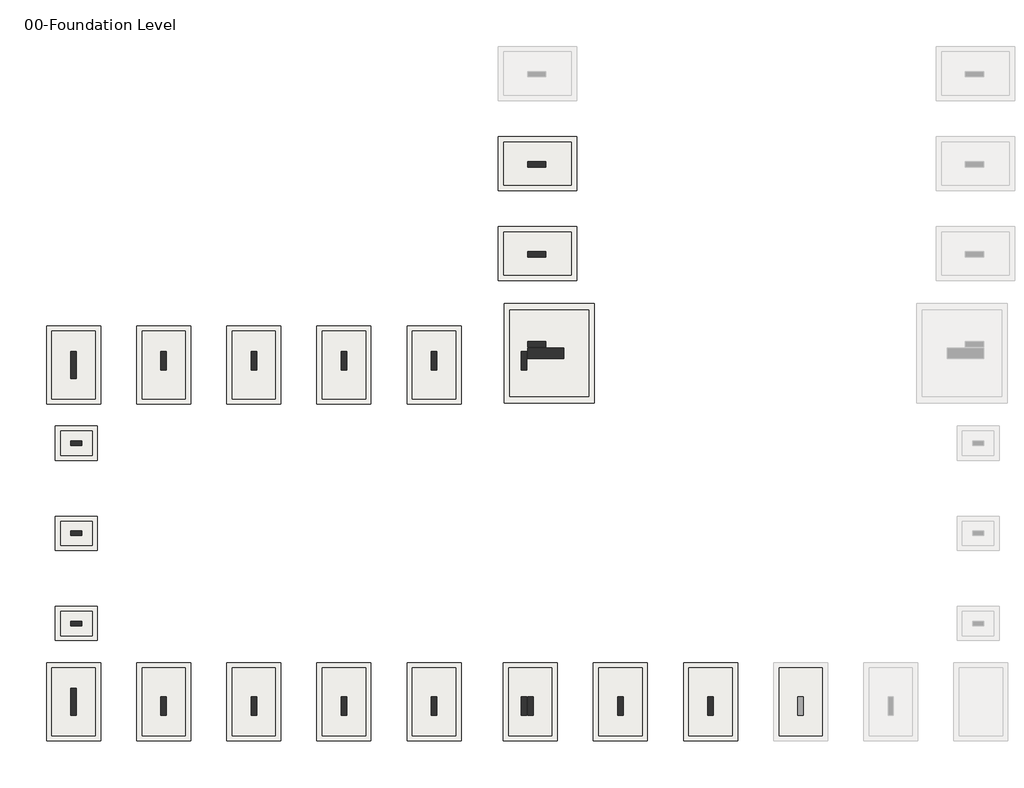
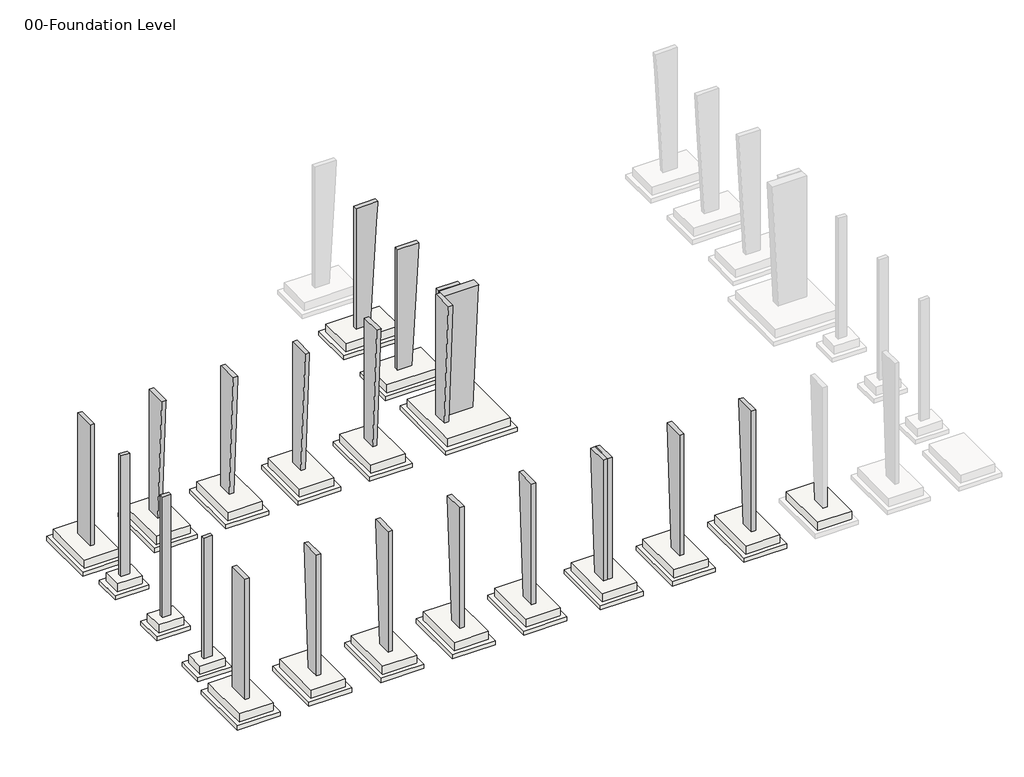
# One storey, part 1 of 4: 39 slabs, 22 columns.
"""IFC4 building model written with IfcOpenShell, lengths in millimetres."""

import ifcopenshell
import ifcopenshell.guid

model = None  # the IFC model being written
_history = None  # IfcOwnerHistory: only IFC2X3 demands one
_inside = {}  # id of a spatial element -> (the spatial element, [elements in it])
_under = {}  # id of a project, library or spatial element -> (it, [spatial elements below it])
_declared = {}  # id of a project -> (the project, [libraries it declares])
_typed = {}  # id of a type object -> (the type object, [elements of that type])
_made_of = {}  # id of a material, layer set ... -> (it, [elements and type objects made of it])


def new_model(schema):
    """Start an empty IFC model of exactly this schema.

    Asked for "IFC4X3", IfcOpenShell would pick the latest addendum, in which some entities
    have other attributes; the version numbers below select the first issue.
    IFC2X3 requires an IfcOwnerHistory on every rooted entity: one is made here for all.
    """
    global model, _history
    if schema == "IFC4X3":
        model = ifcopenshell.file(schema_version=(4, 3, 0, 0))
    else:
        model = ifcopenshell.file(schema=schema)
    _inside.clear()
    _under.clear()
    _declared.clear()
    _typed.clear()
    _made_of.clear()
    _history = None
    if model.schema == "IFC2X3":
        org = make("IfcOrganization", Name="unknown")
        user = make(
            "IfcPersonAndOrganization",
            ThePerson=make("IfcPerson", FamilyName="unknown"),
            TheOrganization=org,
        )
        app = make(
            "IfcApplication",
            ApplicationDeveloper=org,
            Version="unknown",
            ApplicationFullName="unknown",
            ApplicationIdentifier="unknown",
        )
        _history = make(
            "IfcOwnerHistory",
            OwningUser=user,
            OwningApplication=app,
            ChangeAction="ADDED",
            CreationDate=0,
        )
    return model


def make(cls, **values):
    """One entity of the class cls with the attributes given. An attribute that is None is left unset."""
    return model.create_entity(
        cls, **{name: value for name, value in values.items() if value is not None}
    )


def rooted(cls, **values):
    """An entity with a GlobalId (a new one), such as an element, a storey or a relation."""
    return make(cls, GlobalId=ifcopenshell.guid.new(), OwnerHistory=_history, **values)


def si_unit(unit_type, name, prefix=None):
    """IfcSIUnit, for example si_unit("LENGTHUNIT", "METRE", prefix="MILLI")."""
    return make("IfcSIUnit", UnitType=unit_type, Prefix=prefix, Name=name)


def assignment(units):
    """IfcUnitAssignment: the units of a project."""
    return None if units is None else make("IfcUnitAssignment", Units=units)


def point(xyz):
    """IfcCartesianPoint."""
    return None if xyz is None else make("IfcCartesianPoint", Coordinates=xyz)


def direction(xyz):
    """IfcDirection."""
    return None if xyz is None else make("IfcDirection", DirectionRatios=xyz)


def frame(location, z_axis=None, x_axis=None):
    """IfcAxis2Placement3D, a coordinate frame: its origin and axes. An axis left out is left unset."""
    return make(
        "IfcAxis2Placement3D",
        Location=point(location),
        Axis=direction(z_axis),
        RefDirection=direction(x_axis),
    )


def origin():
    """The frame at (0, 0, 0) with its axes left unset."""
    return frame((0.0, 0.0, 0.0))


def place(relative_to, where):
    """IfcLocalPlacement: puts the frame where relative to a parent placement (None: the world)."""
    return make(
        "IfcLocalPlacement", PlacementRelTo=relative_to, RelativePlacement=where
    )


def context(
    kind, dimensions, precision=None, world=None, true_north=None, identifier=None
):
    """IfcGeometricRepresentationContext, for example the 3D "Model" context."""
    return make(
        "IfcGeometricRepresentationContext",
        ContextIdentifier=identifier,
        ContextType=kind,
        CoordinateSpaceDimension=dimensions,
        Precision=precision,
        WorldCoordinateSystem=world,
        TrueNorth=true_north,
    )


def project(units=None, contexts=None):
    """IfcProject with its units and contexts."""
    return rooted(
        "IfcProject",
        Name="project",
        RepresentationContexts=contexts,
        UnitsInContext=assignment(units),
    )


def spatial(cls, under=None, at=None, **own):
    """A site, building, storey or space (cls), placed at a placement, below another one or the project."""
    s = rooted(cls, ObjectPlacement=at, **own)
    if under is not None:
        _under.setdefault(under.id(), (under, []))[1].append(s)
    return s


def polyline(points):
    """IfcPolyline through the points."""
    return make("IfcPolyline", Points=[point(p) for p in points])


def outline(outer, holes=None, kind="AREA"):
    """IfcArbitraryClosedProfileDef: a profile drawn as a closed curve; with holes, ...WithVoids."""
    if holes is None:
        return make("IfcArbitraryClosedProfileDef", ProfileType=kind, OuterCurve=outer)
    return make(
        "IfcArbitraryProfileDefWithVoids",
        ProfileType=kind,
        OuterCurve=outer,
        InnerCurves=holes,
    )


def extrude(swept, where, along, depth):
    """IfcExtrudedAreaSolid: the profile swept, set in the frame where, extruded along a direction by depth."""
    return make(
        "IfcExtrudedAreaSolid",
        SweptArea=swept,
        Position=where,
        ExtrudedDirection=direction(along),
        Depth=depth,
    )


def faces_of(points, faces, orient=None, outer=None):
    """IfcFace entities. A face is a list of loops; a loop is a list of indices into points, from 0.

    orient and outer hold one flag for each loop. By default every Orientation is true, the
    first loop of a face is its IfcFaceOuterBound and the others are IfcFaceBound.
    """
    made = []
    for i, loops in enumerate(faces):
        bounds = []
        for j, loop in enumerate(loops):
            is_outer = j == 0 if outer is None else outer[i][j]
            bounds.append(
                make(
                    "IfcFaceOuterBound" if is_outer else "IfcFaceBound",
                    Bound=make("IfcPolyLoop", Polygon=[points[k] for k in loop]),
                    Orientation=True if orient is None else orient[i][j],
                )
            )
        made.append(make("IfcFace", Bounds=bounds))
    return made


def faceted_brep(points, faces, orient=None, outer=None, voids=None):
    """IfcFacetedBrep: a solid bounded by flat faces; with voids (closed shells), ...WithVoids."""
    shared = [point(p) for p in points]
    hull = make("IfcClosedShell", CfsFaces=faces_of(shared, faces, orient, outer))
    if voids is None:
        return make("IfcFacetedBrep", Outer=hull)
    return make(
        "IfcFacetedBrepWithVoids",
        Outer=hull,
        Voids=[
            make(cls, CfsFaces=faces_of(shared, fs, o, b)) for cls, fs, o, b in voids
        ],
    )


def shape(context_of_items, identifier, shape_type, items):
    """IfcShapeRepresentation: the items that make up one representation, for example the "Body"."""
    return make(
        "IfcShapeRepresentation",
        ContextOfItems=context_of_items,
        RepresentationIdentifier=identifier,
        RepresentationType=shape_type,
        Items=items,
    )


def made_of(thing, what):
    """Note that an element or type object is made of a material, layer set ...; save() writes the relation."""
    if what is not None:
        _made_of.setdefault(what.id(), (what, []))[1].append(thing)
    return thing


def element(
    cls,
    number,
    at=None,
    inside=None,
    cuts=None,
    type_object=None,
    material=None,
    context=None,
    identifier="Body",
    shape_type=None,
    held_by="IfcProductDefinitionShape",
    body=None,
    shapes=None,
    **own,
):
    """One element of the class cls, such as IfcWall. Its Tag is "e" and its number.

    at: its placement. inside: the storey or other place that contains it. cuts: it is an
    opening in that element (IfcRelVoidsElement). A single representation is given by context,
    identifier, shape_type and body (its items); several are given by shapes. held_by: the class
    of the entity that holds the representations. save() writes the other relations.
    """
    e = rooted(cls, Tag="e%d" % number, ObjectPlacement=at, **own)
    if body is not None:
        shapes = [shape(context, identifier, shape_type, body)]
    if shapes is not None:
        e.Representation = make(held_by, Representations=shapes)
    if inside is not None:
        _inside.setdefault(inside.id(), (inside, []))[1].append(e)
    if cuts is not None:
        rooted(
            "IfcRelVoidsElement", RelatingBuildingElement=cuts, RelatedOpeningElement=e
        )
    if type_object is not None:
        _typed.setdefault(type_object.id(), (type_object, []))[1].append(e)
    return made_of(e, material)


def aggregate(whole, parts):
    """IfcRelAggregates: a whole, such as a stair, and the parts it consists of."""
    return rooted("IfcRelAggregates", RelatingObject=whole, RelatedObjects=parts)


def save(model, path):
    """Write the relations noted so far, then the file.

    IfcRelAggregates (storeys below a building ...), IfcRelContainedInSpatialStructure (elements
    in a storey), IfcRelDefinesByType, IfcRelAssociatesMaterial and IfcRelDeclares: one each for
    every whole, place, type object, material and project.
    """
    for whole, parts in _under.values():
        aggregate(whole, parts)
    for where, things in _inside.values():
        rooted(
            "IfcRelContainedInSpatialStructure",
            RelatedElements=things,
            RelatingStructure=where,
        )
    for kind, things in _typed.values():
        rooted("IfcRelDefinesByType", RelatedObjects=things, RelatingType=kind)
    for what, things in _made_of.values():
        rooted("IfcRelAssociatesMaterial", RelatedObjects=things, RelatingMaterial=what)
    for by, libraries in _declared.values():
        rooted("IfcRelDeclares", RelatingContext=by, RelatedDefinitions=libraries)
    model.write(path)


model = new_model("IFC4")

# Units and contexts
model_context = context("Model", 3, world=origin())
ifc_project = project(units=[si_unit("LENGTHUNIT", "METRE", prefix="MILLI")], contexts=[model_context])

# Site, building, storey
site = spatial("IfcSite", under=ifc_project)
building = spatial("IfcBuilding", under=site)
storey = spatial("IfcBuildingStorey", under=building, Name="00-Foundation Level", Elevation=-2000.0)

# Columns
placement = place(None, origin())
element("IfcColumn", 1, ObjectType="Frame Col.2 : 1500x300", at=placement, inside=storey, context=model_context, shape_type="Brep", body=[
    faceted_brep([(25143.2245521, 19099.7448193, -1100.0), (25143.2245521, 20099.7448193, -1100.0), (25143.2245521, 20099.7448193, 7800.0), (25143.2245521, 18599.7448193, 7800.0), (25143.2245521, 18606.4863924, 7680.0), (24843.2245521, 18599.7448193, 7800.0), (24843.2245521, 18606.4863924, 7680.0), (24843.2245521, 19099.7448193, -1100.0), (24843.2245521, 20099.7448193, -1100.0), (24843.2245521, 20089.7085236, 7800.0), (24843.2245521, 20099.7448193, 7800.0)], [[[0, 1, 2, 3, 4]], [[0, 4, 3, 5, 6, 7]], [[8, 7, 6, 5, 9, 10]], [[2, 1, 8, 10]], [[1, 0, 7, 8]], [[3, 2, 10, 9, 5]]]),
])
element("IfcColumn", 2, ObjectType="Frame Col.2 : 1500x300", at=placement, inside=storey, context=model_context, shape_type="Brep", body=[
    faceted_brep([(20143.2245522, 19099.7448193, -1100.0), (20143.2245522, 20099.7448193, -1100.0), (20143.2245522, 20099.7448193, 7800.0), (20143.2245522, 20089.7085236, 7800.0), (20143.2245522, 18599.7448193, 7800.0), (20143.2245522, 18606.4863924, 7680.0), (19843.2245522, 18599.7448193, 7800.0), (19843.2245522, 18606.4863924, 7680.0), (19843.2245522, 19099.7448193, -1100.0), (19843.2245522, 20099.7448193, -1100.0), (19843.2245522, 20089.7085236, 7800.0), (19843.2245522, 20099.7448193, 7800.0)], [[[0, 1, 2, 3, 4, 5]], [[0, 5, 4, 6, 7, 8]], [[9, 8, 7, 6, 10, 11]], [[2, 1, 9, 11]], [[1, 0, 8, 9]], [[4, 3, 2, 11, 10, 6]]]),
])
element("IfcColumn", 3, ObjectType="Frame Col.2 : 1500x300", at=placement, inside=storey, context=model_context, shape_type="Brep", body=[
    faceted_brep([(15143.2245516, 19099.7448193, -1100.0), (15143.2245516, 20099.7448193, -1100.0), (15143.2245516, 20099.7448193, 7800.0), (15143.2245516, 20089.7085236, 7800.0), (15143.2245516, 18599.7448193, 7800.0), (15143.2245516, 18606.4863924, 7680.0), (14843.2245516, 18599.7448193, 7800.0), (14843.2245516, 18606.4863924, 7680.0), (14843.2245516, 19099.7448193, -1100.0), (14843.2245516, 20099.7448193, -1100.0), (14843.2245516, 20089.7085236, 7800.0), (14843.2245516, 20099.7448193, 7800.0)], [[[0, 1, 2, 3, 4, 5]], [[0, 5, 4, 6, 7, 8]], [[9, 8, 7, 6, 10, 11]], [[2, 1, 9, 11]], [[1, 0, 8, 9]], [[4, 3, 2, 11, 10, 6]]]),
])
element("IfcColumn", 4, ObjectType="Frame Col.2 : 1500x300", at=placement, inside=storey, context=model_context, shape_type="Brep", body=[
    faceted_brep([(10143.2245521, 19099.7448193, -1100.0), (10143.2245521, 20099.7448193, -1100.0), (10143.2245521, 20099.7448193, 7800.0), (10143.2245521, 20089.7085236, 7800.0), (10143.2245521, 18599.7448193, 7800.0), (10143.2245521, 18606.4863924, 7680.0), (9843.2245521, 18599.7448193, 7800.0), (9843.2245521, 18606.4863924, 7680.0), (9843.2245521, 19099.7448193, -1100.0), (9843.2245521, 20099.7448193, -1100.0), (9843.2245521, 20089.7085236, 7800.0), (9843.2245521, 20099.7448193, 7800.0)], [[[0, 1, 2, 3, 4, 5]], [[0, 5, 4, 6, 7, 8]], [[9, 8, 7, 6, 10, 11]], [[2, 1, 9, 11]], [[1, 0, 8, 9]], [[4, 3, 2, 11, 10, 6]]]),
])
element("IfcColumn", 5, ObjectType="Frame Col.2 : 1500x300", at=placement, inside=storey, context=model_context, shape_type="Brep", body=[
    faceted_brep([(5143.2245516, 19099.7448193, -1100.0), (5143.2245516, 20099.7448193, -1100.0), (5143.2245516, 20099.7448193, 7800.0), (5143.2245516, 20089.7085236, 7800.0), (5143.2245516, 18599.7448193, 7800.0), (5143.2245516, 18606.4863924, 7680.0), (4843.2245516, 18599.7448193, 7800.0), (4843.2245516, 18606.4863924, 7680.0), (4843.2245516, 19099.7448193, -1100.0), (4843.2245516, 20099.7448193, -1100.0), (4843.2245516, 20089.7085236, 7800.0), (4843.2245516, 20099.7448193, 7800.0)], [[[0, 1, 2, 3, 4, 5]], [[0, 5, 4, 6, 7, 8]], [[9, 8, 7, 6, 10, 11]], [[2, 1, 9, 11]], [[1, 0, 8, 9]], [[4, 3, 2, 11, 10, 6]]]),
])
element("IfcColumn", 6, ObjectType="Frame Col.2 : 1500x300", at=placement, inside=storey, context=model_context, shape_type="Brep", body=[
    faceted_brep([(30183.2245515, 899.7448196, -1100.0), (30183.2245515, -100.2551804, -1100.0), (30183.2245515, -100.2551804, 7680.0), (30183.2245515, -100.2551804, 7800.0), (30183.2245515, 1399.7448196, 7800.0), (30183.2245515, 1393.0032466, 7680.0), (30483.2245515, 1399.7448196, 7800.0), (30483.2245515, 1393.0032466, 7680.0), (30483.2245515, 899.7448196, -1100.0), (30483.2245515, -100.2551804, -1100.0), (30483.2245515, -100.2551804, 7800.0), (30483.2245515, -100.2551804, 7680.0)], [[[0, 1, 2, 3, 4, 5]], [[0, 5, 4, 6, 7, 8]], [[9, 8, 7, 6, 10, 11]], [[3, 2, 1, 9, 11, 10]], [[1, 0, 8, 9]], [[4, 3, 10, 6]]]),
])
element("IfcColumn", 7, ObjectType="Frame Col.2 : 1500x300", at=placement, inside=storey, context=model_context, shape_type="Brep", body=[
    faceted_brep([(25183.2245516, 899.7448196, -1100.0), (25183.2245516, -100.2551804, -1100.0), (25183.2245516, -100.2551804, 7800.0), (25183.2245516, 1399.7448196, 7800.0), (25183.2245516, 1393.0032466, 7680.0), (25483.2245516, 1399.7448196, 7800.0), (25483.2245516, 1393.0032466, 7680.0), (25483.2245516, 899.7448196, -1100.0), (25483.2245516, -100.2551804, -1100.0), (25483.2245516, -100.2551804, 7800.0), (25483.2245516, -100.2551804, 7680.0)], [[[0, 1, 2, 3, 4]], [[0, 4, 3, 5, 6, 7]], [[8, 7, 6, 5, 9, 10]], [[2, 1, 8, 10, 9]], [[1, 0, 7, 8]], [[3, 2, 9, 5]]]),
])
element("IfcColumn", 8, ObjectType="Frame Col.2 : 1500x300", at=placement, inside=storey, context=model_context, shape_type="Brep", body=[
    faceted_brep([(24843.2245521, 899.7448196, -1100.0), (24843.2245521, -100.2551804, -1100.0), (24843.2245521, -100.2551804, 7680.0), (24843.2245521, -100.2551804, 7800.0), (24843.2245521, 1399.7448196, 7800.0), (24843.2245521, 1393.0032466, 7680.0), (25143.2245521, 1399.7448196, 7800.0), (25143.2245521, 1393.0032466, 7680.0), (25143.2245521, 899.7448196, -1100.0), (25143.2245521, -100.2551804, -1100.0), (25143.2245521, -100.2551804, 7800.0), (25143.2245521, -100.2551804, 7680.0)], [[[0, 1, 2, 3, 4, 5]], [[0, 5, 4, 6, 7, 8]], [[9, 8, 7, 6, 10, 11]], [[3, 2, 1, 9, 11, 10]], [[1, 0, 8, 9]], [[4, 3, 10, 6]]]),
])
element("IfcColumn", 9, ObjectType="Frame Col.2 : 1500x300", at=placement, inside=storey, context=model_context, shape_type="Brep", body=[
    faceted_brep([(19843.2245522, 899.7448196, -1100.0), (19843.2245522, -100.2551804, -1100.0), (19843.2245522, -100.2551804, 7680.0), (19843.2245522, -100.2551804, 7800.0), (19843.2245522, 1399.7448196, 7800.0), (19843.2245522, 1393.0032466, 7680.0), (20143.2245522, 1399.7448196, 7800.0), (20143.2245522, 1393.0032466, 7680.0), (20143.2245522, 899.7448196, -1100.0), (20143.2245522, -100.2551804, -1100.0), (20143.2245522, -100.2551804, 7800.0), (20143.2245522, -100.2551804, 7680.0)], [[[0, 1, 2, 3, 4, 5]], [[0, 5, 4, 6, 7, 8]], [[9, 8, 7, 6, 10, 11]], [[3, 2, 1, 9, 11, 10]], [[1, 0, 8, 9]], [[4, 3, 10, 6]]]),
])
element("IfcColumn", 10, ObjectType="Frame Col.2 : 1500x300", at=placement, inside=storey, context=model_context, shape_type="Brep", body=[
    faceted_brep([(14843.2245516, 899.7448196, -1100.0), (14843.2245516, -100.2551804, -1100.0), (14843.2245516, -100.2551804, 7680.0), (14843.2245516, -100.2551804, 7800.0), (14843.2245516, 1399.7448196, 7800.0), (14843.2245516, 1393.0032466, 7680.0), (15143.2245516, 1399.7448196, 7800.0), (15143.2245516, 1393.0032466, 7680.0), (15143.2245516, 899.7448196, -1100.0), (15143.2245516, -100.2551804, -1100.0), (15143.2245516, -100.2551804, 7800.0), (15143.2245516, -100.2551804, 7680.0)], [[[0, 1, 2, 3, 4, 5]], [[0, 5, 4, 6, 7, 8]], [[9, 8, 7, 6, 10, 11]], [[3, 2, 1, 9, 11, 10]], [[1, 0, 8, 9]], [[4, 3, 10, 6]]]),
])
element("IfcColumn", 11, ObjectType="Frame Col.2 : 1500x300", at=placement, inside=storey, context=model_context, shape_type="Brep", body=[
    faceted_brep([(9843.2245521, 899.7448196, -1100.0), (9843.2245521, -100.2551804, -1100.0), (9843.2245521, -100.2551804, 7680.0), (9843.2245521, -100.2551804, 7800.0), (9843.2245521, 1399.7448196, 7800.0), (9843.2245521, 1393.0032466, 7680.0), (10143.2245521, 1399.7448196, 7800.0), (10143.2245521, 1393.0032466, 7680.0), (10143.2245521, 899.7448196, -1100.0), (10143.2245521, -100.2551804, -1100.0), (10143.2245521, -100.2551804, 7800.0), (10143.2245521, -100.2551804, 7680.0)], [[[0, 1, 2, 3, 4, 5]], [[0, 5, 4, 6, 7, 8]], [[9, 8, 7, 6, 10, 11]], [[3, 2, 1, 9, 11, 10]], [[1, 0, 8, 9]], [[4, 3, 10, 6]]]),
])
element("IfcColumn", 12, ObjectType="Frame Col.2 : 1500x300", at=placement, inside=storey, context=model_context, shape_type="Brep", body=[
    faceted_brep([(4843.2245516, 899.7448196, -1100.0), (4843.2245516, -100.2551804, -1100.0), (4843.2245516, -100.2551804, 7680.0), (4843.2245516, -100.2551804, 7800.0), (4843.2245516, 1399.7448196, 7800.0), (4843.2245516, 1393.0032466, 7680.0), (5143.2245516, 1399.7448196, 7800.0), (5143.2245516, 1393.0032466, 7680.0), (5143.2245516, 899.7448196, -1100.0), (5143.2245516, -100.2551804, -1100.0), (5143.2245516, -100.2551804, 7800.0), (5143.2245516, -100.2551804, 7680.0)], [[[0, 1, 2, 3, 4, 5]], [[0, 5, 4, 6, 7, 8]], [[9, 8, 7, 6, 10, 11]], [[3, 2, 1, 9, 11, 10]], [[1, 0, 8, 9]], [[4, 3, 10, 6]]]),
])
element("IfcColumn", 13, ObjectType="Frame Col.2 : 1500x300", at=placement, inside=storey, context=model_context, shape_type="Brep", body=[
    faceted_brep([(26183.2245516, 20639.9999998, -1100.0), (25183.2245516, 20639.9999998, -1100.0), (25183.2245516, 20639.9999998, 7680.0), (25183.2245516, 20639.9999998, 7800.0), (26683.2245516, 20639.9999998, 7800.0), (26676.4829785, 20639.9999998, 7680.0), (26683.2245516, 20339.9999998, 7800.0), (26676.4829785, 20339.9999998, 7680.0), (26183.2245516, 20339.9999998, -1100.0), (25183.2245516, 20339.9999998, -1100.0), (25183.2245516, 20339.9999998, 7800.0)], [[[0, 1, 2, 3, 4, 5]], [[0, 5, 4, 6, 7, 8]], [[9, 8, 7, 6, 10]], [[3, 2, 1, 9, 10]], [[1, 0, 8, 9]], [[4, 3, 10, 6]]]),
])
element("IfcColumn", 14, ObjectType="Frame Col.2 : 1500x300", at=placement, inside=storey, context=model_context, shape_type="Brep", body=[
    faceted_brep([(35183.2245515, 899.7448196, -1100.0), (35183.2245515, -100.2551804, -1100.0), (35183.2245515, -100.2551804, 7680.0), (35183.2245515, -100.2551804, 7800.0), (35183.2245515, 1399.7448196, 7800.0), (35183.2245515, 1393.0032466, 7680.0), (35483.2245515, 1399.7448196, 7800.0), (35483.2245515, 1393.0032466, 7680.0), (35483.2245515, 899.7448196, -1100.0), (35483.2245515, -100.2551804, -1100.0), (35483.2245515, -100.2551804, 7800.0), (35483.2245515, -100.2551804, 7680.0)], [[[0, 1, 2, 3, 4, 5]], [[0, 5, 4, 6, 7, 8]], [[9, 8, 7, 6, 10, 11]], [[3, 2, 1, 9, 11, 10]], [[1, 0, 8, 9]], [[4, 3, 10, 6]]]),
])
element("IfcColumn", 15, ObjectType="Frame Col.2 : 1500x300", at=placement, inside=storey, context=model_context, shape_type="Brep", body=[
    faceted_brep([(26183.2245516, 25639.9999988, -1100.0), (25183.2245516, 25639.9999988, -1100.0), (25183.2245516, 25639.9999988, 7680.0), (25183.2245516, 25639.9999988, 7800.0), (26683.2245516, 25639.9999988, 7800.0), (26676.4829785, 25639.9999988, 7680.0), (26598.9548887, 25639.9999988, 6300.0), (26683.2245516, 25339.9999988, 7800.0), (26676.4829785, 25339.9999988, 7680.0), (26598.9548887, 25339.9999988, 6300.0), (26183.2245516, 25339.9999988, -1100.0), (25183.2245516, 25339.9999988, -1100.0), (25183.2245516, 25339.9999988, 7800.0), (25183.2245516, 25339.9999988, 7680.0)], [[[0, 1, 2, 3, 4, 5, 6]], [[0, 6, 5, 4, 7, 8, 9, 10]], [[11, 10, 9, 8, 7, 12, 13]], [[3, 2, 1, 11, 13, 12]], [[1, 0, 10, 11]], [[4, 3, 12, 7]]]),
])
element("IfcColumn", 16, ObjectType="Frame Col.2 : 1500x300", at=placement, inside=storey, context=model_context, shape_type="Brep", body=[
    faceted_brep([(26183.2245516, 30639.9999988, -1100.0), (25183.2245516, 30639.9999988, -1100.0), (25183.2245516, 30639.9999988, 7680.0), (25183.2245516, 30639.9999988, 7800.0), (26683.2245516, 30639.9999988, 7800.0), (26676.4829785, 30639.9999988, 7680.0), (26598.9548887, 30639.9999988, 6300.0), (26683.2245516, 30339.9999988, 7800.0), (26676.4829785, 30339.9999988, 7680.0), (26598.9548887, 30339.9999988, 6300.0), (26183.2245516, 30339.9999988, -1100.0), (25183.2245516, 30339.9999988, -1100.0), (25183.2245516, 30339.9999988, 7800.0), (25183.2245516, 30339.9999988, 7680.0)], [[[0, 1, 2, 3, 4, 5, 6]], [[0, 6, 5, 4, 7, 8, 9, 10]], [[11, 10, 9, 8, 7, 12, 13]], [[3, 2, 1, 11, 13, 12]], [[1, 0, 10, 11]], [[4, 3, 12, 7]]]),
])
element("IfcColumn", 17, ObjectType="Frame Col.2 : 2400x600", at=placement, inside=storey, context=model_context, shape_type="Brep", body=[
    faceted_brep([(27183.2245516, 20299.9999995, -1100.0), (25183.2245516, 20299.9999995, -1100.0), (25183.2245516, 20299.9999995, 7800.0), (27583.2245516, 20299.9999995, 7800.0), (27577.8312932, 20299.9999995, 7680.0), (27583.2245516, 19699.9999995, 7800.0), (27577.8312932, 19699.9999995, 7680.0), (27183.2245516, 19699.9999995, -1100.0), (25183.2245516, 19699.9999995, -1100.0), (25183.2245516, 19699.9999995, 7800.0), (25183.2245516, 19699.9999995, 7680.0)], [[[0, 1, 2, 3, 4]], [[0, 4, 3, 5, 6, 7]], [[8, 7, 6, 5, 9, 10]], [[2, 1, 8, 10, 9]], [[1, 0, 7, 8]], [[3, 2, 9, 5]]]),
])
element("IfcColumn", 18, ObjectType="M_Concrete-Rectangular-Column : 250 x 600mm", at=placement, inside=storey, context=model_context, shape_type="Brep", body=[
    faceted_brep([(-156.7754479, 15124.9999995, -1100.0), (443.2245521, 15124.9999995, -1100.0), (443.2245521, 14874.9999995, -1100.0), (-156.7754479, 14874.9999995, -1100.0), (-156.7754479, 15124.9999995, 7680.0), (-156.7754479, 15124.9999995, 7800.0), (443.2245521, 15124.9999995, 7800.0), (443.2245521, 15124.9999995, 7680.0), (-156.7754479, 14874.9999995, 7680.0), (-156.7754479, 14874.9999995, 7800.0), (443.2245521, 14874.9999995, 7680.0), (443.2245521, 14874.9999995, 7800.0)], [[[0, 1, 2, 3]], [[1, 0, 4, 5, 6, 7]], [[0, 3, 8, 9, 5, 4]], [[3, 2, 10, 11, 9, 8]], [[2, 1, 7, 6, 11, 10]], [[6, 5, 9, 11]]]),
])
element("IfcColumn", 19, ObjectType="M_Concrete-Rectangular-Column : 250 x 600mm", at=placement, inside=storey, context=model_context, shape_type="Brep", body=[
    faceted_brep([(-156.7754479, 10124.9999995, -1100.0), (443.2245521, 10124.9999995, -1100.0), (443.2245521, 9874.9999995, -1100.0), (-156.7754479, 9874.9999995, -1100.0), (-156.7754479, 10124.9999995, 7680.0), (-156.7754479, 10124.9999995, 7800.0), (443.2245521, 10124.9999995, 7800.0), (443.2245521, 10124.9999995, 7680.0), (-156.7754479, 9874.9999995, 7680.0), (-156.7754479, 9874.9999995, 7800.0), (443.2245521, 9874.9999995, 7680.0), (443.2245521, 9874.9999995, 7800.0)], [[[0, 1, 2, 3]], [[1, 0, 4, 5, 6, 7]], [[0, 3, 8, 9, 5, 4]], [[3, 2, 10, 11, 9, 8]], [[2, 1, 7, 6, 11, 10]], [[6, 5, 9, 11]]]),
])
element("IfcColumn", 20, ObjectType="M_Concrete-Rectangular-Column : 250 x 600mm", at=placement, inside=storey, context=model_context, shape_type="Brep", body=[
    faceted_brep([(-156.7754479, 5124.9999995, -1100.0), (443.2245521, 5124.9999995, -1100.0), (443.2245521, 4874.9999995, -1100.0), (-156.7754479, 4874.9999995, -1100.0), (-156.7754479, 5124.9999995, 7680.0), (-156.7754479, 5124.9999995, 7800.0), (443.2245521, 5124.9999995, 7800.0), (443.2245521, 5124.9999995, 7680.0), (-156.7754479, 4874.9999995, 7680.0), (-156.7754479, 4874.9999995, 7800.0), (443.2245521, 4874.9999995, 7680.0), (443.2245521, 4874.9999995, 7800.0)], [[[0, 1, 2, 3]], [[1, 0, 4, 5, 6, 7]], [[0, 3, 8, 9, 5, 4]], [[3, 2, 10, 11, 9, 8]], [[2, 1, 7, 6, 11, 10]], [[6, 5, 9, 11]]]),
])
element("IfcColumn", 21, ObjectType="M_Concrete-Rectangular-Column : 300 x 1500mm", at=placement, inside=storey, context=model_context, shape_type="Brep", body=[
    faceted_brep([(-156.7754479, 18599.7448193, -1100.0), (-156.7754479, 20099.7448193, -1100.0), (143.2245521, 20099.7448193, -1100.0), (143.2245521, 18599.7448193, -1100.0), (-156.7754479, 18599.7448193, 7680.0), (-156.7754479, 18599.7448193, 7800.0), (-156.7754479, 20099.7448193, 7800.0), (143.2245521, 18599.7448193, 7680.0), (143.2245521, 18599.7448193, 7800.0), (143.2245521, 20099.7448193, 7800.0), (143.2245521, 20089.7085236, 7800.0)], [[[0, 1, 2, 3]], [[1, 0, 4, 5, 6]], [[0, 3, 7, 8, 5, 4]], [[3, 2, 9, 10, 8, 7]], [[2, 1, 6, 9]], [[6, 5, 8, 10, 9]]]),
])
element("IfcColumn", 22, ObjectType="M_Concrete-Rectangular-Column : 300 x 1500mm", at=placement, inside=storey, context=model_context, shape_type="Brep", body=[
    faceted_brep([(-156.7754479, -100.2551804, -1100.0), (-156.7754479, 1399.7448196, -1100.0), (143.2245521, 1399.7448196, -1100.0), (143.2245521, -100.2551804, -1100.0), (-156.7754479, -100.2551804, 7680.0), (-156.7754479, -100.2551804, 7800.0), (-156.7754479, 1399.7448196, 7800.0), (-156.7754479, 1399.7448196, 7680.0), (143.2245521, -100.2551804, 7680.0), (143.2245521, -100.2551804, 7800.0), (143.2245521, 1399.7448196, 7680.0), (143.2245521, 1399.7448196, 7800.0)], [[[0, 1, 2, 3]], [[1, 0, 4, 5, 6, 7]], [[0, 3, 8, 9, 5, 4]], [[3, 2, 10, 11, 9, 8]], [[2, 1, 7, 6, 11, 10]], [[6, 5, 9, 11]]]),
])

# Slabs
element("IfcSlab", 23, ObjectType="M_Footing-Rectangular : PC 2-2350 x 1900 x 300mm", at=placement, inside=storey, context=model_context, shape_type="SweptSolid", body=[
    extrude(outline(polyline([(1318.2245521, 15949.9999995), (1318.2245521, 14049.9999995), (-1031.7754479, 14049.9999995), (-1031.7754479, 15949.9999995), (1318.2245521, 15949.9999995)])), frame((0.0, 0.0, -2000.0), z_axis=(0.0, 0.0, 1.0), x_axis=(1.0, 0.0, 0.0)), (0.0, 0.0, 1.0), 300.0),
])
element("IfcSlab", 24, ObjectType="M_Footing-Rectangular : PC 2-2350 x 1900 x 300mm", at=placement, inside=storey, context=model_context, shape_type="SweptSolid", body=[
    extrude(outline(polyline([(1318.2245521, 10949.9999995), (1318.2245521, 9049.9999995), (-1031.7754479, 9049.9999995), (-1031.7754479, 10949.9999995), (1318.2245521, 10949.9999995)])), frame((0.0, 0.0, -2000.0), z_axis=(0.0, 0.0, 1.0), x_axis=(1.0, 0.0, 0.0)), (0.0, 0.0, 1.0), 300.0),
])
element("IfcSlab", 25, ObjectType="M_Footing-Rectangular : PC 2-2350 x 1900 x 300mm", at=placement, inside=storey, context=model_context, shape_type="SweptSolid", body=[
    extrude(outline(polyline([(1318.2245521, 5949.9999995), (1318.2245521, 4049.9999995), (-1031.7754479, 4049.9999995), (-1031.7754479, 5949.9999995), (1318.2245521, 5949.9999995)])), frame((0.0, 0.0, -2000.0), z_axis=(0.0, 0.0, 1.0), x_axis=(1.0, 0.0, 0.0)), (0.0, 0.0, 1.0), 300.0),
])
element("IfcSlab", 26, ObjectType="M_Footing-Rectangular : PC 3-5500 x 5000 x 300mm", at=placement, inside=storey, context=model_context, shape_type="SweptSolid", body=[
    extrude(outline(polyline([(23883.2245516, 22749.9999993), (28883.2245516, 22749.9999993), (28883.2245516, 17249.9999993), (23883.2245516, 17249.9999993), (23883.2245516, 22749.9999993)])), frame((0.0, 0.0, -2000.0), z_axis=(0.0, 0.0, 1.0), x_axis=(1.0, 0.0, 0.0)), (0.0, 0.0, 1.0), 300.0),
])
element("IfcSlab", 27, ObjectType="M_Footing-Rectangular : PC-4350 x 3000 x 300mm", at=placement, inside=storey, context=model_context, shape_type="SweptSolid", body=[
    extrude(outline(polyline([(36833.2245515, 2825.0), (36833.2245515, -1525.0), (33833.2245515, -1525.0), (33833.2245515, 2825.0), (36833.2245515, 2825.0)])), frame((0.0, 0.0, -2000.0), z_axis=(0.0, 0.0, 1.0), x_axis=(1.0, 0.0, 0.0)), (0.0, 0.0, 1.0), 300.0),
])
element("IfcSlab", 28, ObjectType="M_Footing-Rectangular : PC-4350 x 3000 x 300mm", at=placement, inside=storey, context=model_context, shape_type="SweptSolid", body=[
    extrude(outline(polyline([(31833.2245515, 2825.0), (31833.2245515, -1525.0), (28833.2245515, -1525.0), (28833.2245515, 2825.0), (31833.2245515, 2825.0)])), frame((0.0, 0.0, -2000.0), z_axis=(0.0, 0.0, 1.0), x_axis=(1.0, 0.0, 0.0)), (0.0, 0.0, 1.0), 300.0),
])
element("IfcSlab", 29, ObjectType="M_Footing-Rectangular : PC-4350 x 3000 x 300mm", at=placement, inside=storey, context=model_context, shape_type="SweptSolid", body=[
    extrude(outline(polyline([(21493.2245522, 2825.0), (21493.2245522, -1525.0), (18493.2245522, -1525.0), (18493.2245522, 2825.0), (21493.2245522, 2825.0)])), frame((0.0, 0.0, -2000.0), z_axis=(0.0, 0.0, 1.0), x_axis=(1.0, 0.0, 0.0)), (0.0, 0.0, 1.0), 300.0),
])
element("IfcSlab", 30, ObjectType="M_Footing-Rectangular : PC-4350 x 3000 x 300mm", at=placement, inside=storey, context=model_context, shape_type="SweptSolid", body=[
    extrude(outline(polyline([(16493.2245516, 2825.0), (16493.2245516, -1525.0), (13493.2245516, -1525.0), (13493.2245516, 2825.0), (16493.2245516, 2825.0)])), frame((0.0, 0.0, -2000.0), z_axis=(0.0, 0.0, 1.0), x_axis=(1.0, 0.0, 0.0)), (0.0, 0.0, 1.0), 300.0),
])
element("IfcSlab", 31, ObjectType="M_Footing-Rectangular : PC-4350 x 3000 x 300mm", at=placement, inside=storey, context=model_context, shape_type="SweptSolid", body=[
    extrude(outline(polyline([(11493.2245521, 2825.0), (11493.2245521, -1525.0), (8493.2245521, -1525.0), (8493.2245521, 2825.0), (11493.2245521, 2825.0)])), frame((0.0, 0.0, -2000.0), z_axis=(0.0, 0.0, 1.0), x_axis=(1.0, 0.0, 0.0)), (0.0, 0.0, 1.0), 300.0),
])
element("IfcSlab", 32, ObjectType="M_Footing-Rectangular : PC-4350 x 3000 x 300mm", at=placement, inside=storey, context=model_context, shape_type="SweptSolid", body=[
    extrude(outline(polyline([(6493.2245516, 2825.0), (6493.2245516, -1525.0), (3493.2245516, -1525.0), (3493.2245516, 2825.0), (6493.2245516, 2825.0)])), frame((0.0, 0.0, -2000.0), z_axis=(0.0, 0.0, 1.0), x_axis=(1.0, 0.0, 0.0)), (0.0, 0.0, 1.0), 300.0),
])
element("IfcSlab", 33, ObjectType="M_Footing-Rectangular : PC-4350 x 3000 x 300mm", at=placement, inside=storey, context=model_context, shape_type="SweptSolid", body=[
    extrude(outline(polyline([(1493.2245521, 2825.0), (1493.2245521, -1525.0), (-1506.7754479, -1525.0), (-1506.7754479, 2825.0), (1493.2245521, 2825.0)])), frame((0.0, 0.0, -2000.0), z_axis=(0.0, 0.0, 1.0), x_axis=(1.0, 0.0, 0.0)), (0.0, 0.0, 1.0), 300.0),
])
element("IfcSlab", 34, ObjectType="M_Footing-Rectangular : PC-4350 x 3000 x 300mm", at=placement, inside=storey, context=model_context, shape_type="SweptSolid", body=[
    extrude(outline(polyline([(21493.2245522, 21525.0000002), (21493.2245522, 17175.0000002), (18493.2245522, 17175.0000002), (18493.2245522, 21525.0000002), (21493.2245522, 21525.0000002)])), frame((0.0, 0.0, -2000.0), z_axis=(0.0, 0.0, 1.0), x_axis=(1.0, 0.0, 0.0)), (0.0, 0.0, 1.0), 300.0),
])
element("IfcSlab", 35, ObjectType="M_Footing-Rectangular : PC-4350 x 3000 x 300mm", at=placement, inside=storey, context=model_context, shape_type="SweptSolid", body=[
    extrude(outline(polyline([(16493.2245516, 21525.0000002), (16493.2245516, 17175.0000002), (13493.2245516, 17175.0000002), (13493.2245516, 21525.0000002), (16493.2245516, 21525.0000002)])), frame((0.0, 0.0, -2000.0), z_axis=(0.0, 0.0, 1.0), x_axis=(1.0, 0.0, 0.0)), (0.0, 0.0, 1.0), 300.0),
])
element("IfcSlab", 36, ObjectType="M_Footing-Rectangular : PC-4350 x 3000 x 300mm", at=placement, inside=storey, context=model_context, shape_type="SweptSolid", body=[
    extrude(outline(polyline([(11493.2245521, 21525.0000002), (11493.2245521, 17175.0000002), (8493.2245521, 17175.0000002), (8493.2245521, 21525.0000002), (11493.2245521, 21525.0000002)])), frame((0.0, 0.0, -2000.0), z_axis=(0.0, 0.0, 1.0), x_axis=(1.0, 0.0, 0.0)), (0.0, 0.0, 1.0), 300.0),
])
element("IfcSlab", 37, ObjectType="M_Footing-Rectangular : PC-4350 x 3000 x 300mm", at=placement, inside=storey, context=model_context, shape_type="SweptSolid", body=[
    extrude(outline(polyline([(6493.2245516, 21525.0000002), (6493.2245516, 17175.0000002), (3493.2245516, 17175.0000002), (3493.2245516, 21525.0000002), (6493.2245516, 21525.0000002)])), frame((0.0, 0.0, -2000.0), z_axis=(0.0, 0.0, 1.0), x_axis=(1.0, 0.0, 0.0)), (0.0, 0.0, 1.0), 300.0),
])
element("IfcSlab", 38, ObjectType="M_Footing-Rectangular : PC-4350 x 3000 x 300mm", at=placement, inside=storey, context=model_context, shape_type="SweptSolid", body=[
    extrude(outline(polyline([(1493.2245521, 21525.0000002), (1493.2245521, 17175.0000002), (-1506.7754479, 17175.0000002), (-1506.7754479, 21525.0000002), (1493.2245521, 21525.0000002)])), frame((0.0, 0.0, -2000.0), z_axis=(0.0, 0.0, 1.0), x_axis=(1.0, 0.0, 0.0)), (0.0, 0.0, 1.0), 300.0),
])
element("IfcSlab", 39, ObjectType="M_Footing-Rectangular : PC-4350 x 3000 x 300mm", at=placement, inside=storey, context=model_context, shape_type="SweptSolid", body=[
    extrude(outline(polyline([(26833.2245516, 2825.0), (26833.2245516, -1525.0), (23833.2245516, -1525.0), (23833.2245516, 2825.0), (26833.2245516, 2825.0)])), frame((0.0, 0.0, -2000.0), z_axis=(0.0, 0.0, 1.0), x_axis=(1.0, 0.0, 0.0)), (0.0, 0.0, 1.0), 300.0),
])
element("IfcSlab", 40, ObjectType="M_Footing-Rectangular : PC-4350 x 3000 x 300mm", at=placement, inside=storey, context=model_context, shape_type="SweptSolid", body=[
    extrude(outline(polyline([(23564.9999997, 32029.7448203), (27914.9999997, 32029.7448203), (27914.9999997, 29029.7448203), (23564.9999997, 29029.7448203), (23564.9999997, 32029.7448203)])), frame((0.0, 0.0, -2000.0), z_axis=(0.0, 0.0, 1.0), x_axis=(1.0, 0.0, 0.0)), (0.0, 0.0, 1.0), 300.0),
])
element("IfcSlab", 41, ObjectType="M_Footing-Rectangular : PC-4350 x 3000 x 300mm", at=placement, inside=storey, context=model_context, shape_type="SweptSolid", body=[
    extrude(outline(polyline([(23564.9999997, 27029.7448203), (27914.9999997, 27029.7448203), (27914.9999997, 24029.7448203), (23564.9999997, 24029.7448203), (23564.9999997, 27029.7448203)])), frame((0.0, 0.0, -2000.0), z_axis=(0.0, 0.0, 1.0), x_axis=(1.0, 0.0, 0.0)), (0.0, 0.0, 1.0), 300.0),
])
element("IfcSlab", 42, ObjectType="M_Footing-Rectangular : RC 2-1750 x 1350 x 600mm", at=placement, inside=storey, context=model_context, shape_type="SweptSolid", body=[
    extrude(outline(polyline([(1018.2245521, 15674.9999995), (1018.2245521, 14324.9999995), (-731.7754479, 14324.9999995), (-731.7754479, 15674.9999995), (1018.2245521, 15674.9999995)])), frame((0.0, 0.0, -1700.0), z_axis=(0.0, 0.0, 1.0), x_axis=(1.0, 0.0, 0.0)), (0.0, 0.0, 1.0), 600.0),
])
element("IfcSlab", 43, ObjectType="M_Footing-Rectangular : RC 2-1750 x 1350 x 600mm", at=placement, inside=storey, context=model_context, shape_type="SweptSolid", body=[
    extrude(outline(polyline([(1018.2245521, 10674.9999995), (1018.2245521, 9324.9999995), (-731.7754479, 9324.9999995), (-731.7754479, 10674.9999995), (1018.2245521, 10674.9999995)])), frame((0.0, 0.0, -1700.0), z_axis=(0.0, 0.0, 1.0), x_axis=(1.0, 0.0, 0.0)), (0.0, 0.0, 1.0), 600.0),
])
element("IfcSlab", 44, ObjectType="M_Footing-Rectangular : RC 2-1750 x 1350 x 600mm", at=placement, inside=storey, context=model_context, shape_type="SweptSolid", body=[
    extrude(outline(polyline([(1018.2245521, 5674.9999995), (1018.2245521, 4324.9999995), (-731.7754479, 4324.9999995), (-731.7754479, 5674.9999995), (1018.2245521, 5674.9999995)])), frame((0.0, 0.0, -1700.0), z_axis=(0.0, 0.0, 1.0), x_axis=(1.0, 0.0, 0.0)), (0.0, 0.0, 1.0), 600.0),
])
element("IfcSlab", 45, ObjectType="M_Footing-Rectangular : RC 3- 4800 x 4400 x 600mm 2", at=placement, inside=storey, context=model_context, shape_type="SweptSolid", body=[
    extrude(outline(polyline([(24183.2245516, 22399.9999993), (28583.2245516, 22399.9999993), (28583.2245516, 17599.9999993), (24183.2245516, 17599.9999993), (24183.2245516, 22399.9999993)])), frame((0.0, 0.0, -1700.0), z_axis=(0.0, 0.0, 1.0), x_axis=(1.0, 0.0, 0.0)), (0.0, 0.0, 1.0), 600.0),
])
element("IfcSlab", 46, ObjectType="M_Footing-Rectangular : RC-3750 x 2400 x 600mm", at=placement, inside=storey, context=model_context, shape_type="SweptSolid", body=[
    extrude(outline(polyline([(41533.2245515, 2525.0), (41533.2245515, -1225.0), (39133.2245515, -1225.0), (39133.2245515, 2525.0), (41533.2245515, 2525.0)])), frame((0.0, 0.0, -1700.0), z_axis=(0.0, 0.0, 1.0), x_axis=(1.0, 0.0, 0.0)), (0.0, 0.0, 1.0), 600.0),
])
element("IfcSlab", 47, ObjectType="M_Footing-Rectangular : RC-3750 x 2400 x 600mm", at=placement, inside=storey, context=model_context, shape_type="SweptSolid", body=[
    extrude(outline(polyline([(36533.2245515, 2525.0), (36533.2245515, -1225.0), (34133.2245515, -1225.0), (34133.2245515, 2525.0), (36533.2245515, 2525.0)])), frame((0.0, 0.0, -1700.0), z_axis=(0.0, 0.0, 1.0), x_axis=(1.0, 0.0, 0.0)), (0.0, 0.0, 1.0), 600.0),
])
element("IfcSlab", 48, ObjectType="M_Footing-Rectangular : RC-3750 x 2400 x 600mm", at=placement, inside=storey, context=model_context, shape_type="SweptSolid", body=[
    extrude(outline(polyline([(31533.2245515, 2525.0), (31533.2245515, -1225.0), (29133.2245515, -1225.0), (29133.2245515, 2525.0), (31533.2245515, 2525.0)])), frame((0.0, 0.0, -1700.0), z_axis=(0.0, 0.0, 1.0), x_axis=(1.0, 0.0, 0.0)), (0.0, 0.0, 1.0), 600.0),
])
element("IfcSlab", 49, ObjectType="M_Footing-Rectangular : RC-3750 x 2400 x 600mm", at=placement, inside=storey, context=model_context, shape_type="SweptSolid", body=[
    extrude(outline(polyline([(21193.224552, 21225.0000002), (21193.224552, 17475.0000002), (18793.224552, 17475.0000002), (18793.224552, 21225.0000002), (21193.224552, 21225.0000002)])), frame((0.0, 0.0, -1700.0), z_axis=(0.0, 0.0, 1.0), x_axis=(1.0, 0.0, 0.0)), (0.0, 0.0, 1.0), 600.0),
])
element("IfcSlab", 50, ObjectType="M_Footing-Rectangular : RC-3750 x 2400 x 600mm", at=placement, inside=storey, context=model_context, shape_type="SweptSolid", body=[
    extrude(outline(polyline([(16193.2245516, 21225.0000002), (16193.2245516, 17475.0000002), (13793.2245516, 17475.0000002), (13793.2245516, 21225.0000002), (16193.2245516, 21225.0000002)])), frame((0.0, 0.0, -1700.0), z_axis=(0.0, 0.0, 1.0), x_axis=(1.0, 0.0, 0.0)), (0.0, 0.0, 1.0), 600.0),
])
element("IfcSlab", 51, ObjectType="M_Footing-Rectangular : RC-3750 x 2400 x 600mm", at=placement, inside=storey, context=model_context, shape_type="SweptSolid", body=[
    extrude(outline(polyline([(11193.224552, 21225.0000002), (11193.224552, 17475.0000002), (8793.224552, 17475.0000002), (8793.224552, 21225.0000002), (11193.224552, 21225.0000002)])), frame((0.0, 0.0, -1700.0), z_axis=(0.0, 0.0, 1.0), x_axis=(1.0, 0.0, 0.0)), (0.0, 0.0, 1.0), 600.0),
])
element("IfcSlab", 52, ObjectType="M_Footing-Rectangular : RC-3750 x 2400 x 600mm", at=placement, inside=storey, context=model_context, shape_type="SweptSolid", body=[
    extrude(outline(polyline([(6193.2245516, 21225.0000002), (6193.2245516, 17475.0000002), (3793.2245516, 17475.0000002), (3793.2245516, 21225.0000002), (6193.2245516, 21225.0000002)])), frame((0.0, 0.0, -1700.0), z_axis=(0.0, 0.0, 1.0), x_axis=(1.0, 0.0, 0.0)), (0.0, 0.0, 1.0), 600.0),
])
element("IfcSlab", 53, ObjectType="M_Footing-Rectangular : RC-3750 x 2400 x 600mm", at=placement, inside=storey, context=model_context, shape_type="SweptSolid", body=[
    extrude(outline(polyline([(21193.224552, 2525.0), (21193.224552, -1225.0), (18793.224552, -1225.0), (18793.224552, 2525.0), (21193.224552, 2525.0)])), frame((0.0, 0.0, -1700.0), z_axis=(0.0, 0.0, 1.0), x_axis=(1.0, 0.0, 0.0)), (0.0, 0.0, 1.0), 600.0),
])
element("IfcSlab", 54, ObjectType="M_Footing-Rectangular : RC-3750 x 2400 x 600mm", at=placement, inside=storey, context=model_context, shape_type="SweptSolid", body=[
    extrude(outline(polyline([(16193.2245516, 2525.0), (16193.2245516, -1225.0), (13793.2245516, -1225.0), (13793.2245516, 2525.0), (16193.2245516, 2525.0)])), frame((0.0, 0.0, -1700.0), z_axis=(0.0, 0.0, 1.0), x_axis=(1.0, 0.0, 0.0)), (0.0, 0.0, 1.0), 600.0),
])
element("IfcSlab", 55, ObjectType="M_Footing-Rectangular : RC-3750 x 2400 x 600mm", at=placement, inside=storey, context=model_context, shape_type="SweptSolid", body=[
    extrude(outline(polyline([(11193.224552, 2525.0), (11193.224552, -1225.0), (8793.224552, -1225.0), (8793.224552, 2525.0), (11193.224552, 2525.0)])), frame((0.0, 0.0, -1700.0), z_axis=(0.0, 0.0, 1.0), x_axis=(1.0, 0.0, 0.0)), (0.0, 0.0, 1.0), 600.0),
])
element("IfcSlab", 56, ObjectType="M_Footing-Rectangular : RC-3750 x 2400 x 600mm", at=placement, inside=storey, context=model_context, shape_type="SweptSolid", body=[
    extrude(outline(polyline([(6193.2245516, 2525.0), (6193.2245516, -1225.0), (3793.2245516, -1225.0), (3793.2245516, 2525.0), (6193.2245516, 2525.0)])), frame((0.0, 0.0, -1700.0), z_axis=(0.0, 0.0, 1.0), x_axis=(1.0, 0.0, 0.0)), (0.0, 0.0, 1.0), 600.0),
])
element("IfcSlab", 57, ObjectType="M_Footing-Rectangular : RC-3750 x 2400 x 600mm", at=placement, inside=storey, context=model_context, shape_type="SweptSolid", body=[
    extrude(outline(polyline([(1193.224552, 21225.0000002), (1193.224552, 17475.0000002), (-1206.775448, 17475.0000002), (-1206.775448, 21225.0000002), (1193.224552, 21225.0000002)])), frame((0.0, 0.0, -1700.0), z_axis=(0.0, 0.0, 1.0), x_axis=(1.0, 0.0, 0.0)), (0.0, 0.0, 1.0), 600.0),
])
element("IfcSlab", 58, ObjectType="M_Footing-Rectangular : RC-3750 x 2400 x 600mm", at=placement, inside=storey, context=model_context, shape_type="SweptSolid", body=[
    extrude(outline(polyline([(1193.2245521, 2525.0), (1193.2245521, -1225.0), (-1206.7754479, -1225.0), (-1206.7754479, 2525.0), (1193.2245521, 2525.0)])), frame((0.0, 0.0, -1700.0), z_axis=(0.0, 0.0, 1.0), x_axis=(1.0, 0.0, 0.0)), (0.0, 0.0, 1.0), 600.0),
])
element("IfcSlab", 59, ObjectType="M_Footing-Rectangular : RC-3750 x 2400 x 600mm", at=placement, inside=storey, context=model_context, shape_type="SweptSolid", body=[
    extrude(outline(polyline([(26533.2245516, 2525.0), (26533.2245516, -1225.0), (24133.2245516, -1225.0), (24133.2245516, 2525.0), (26533.2245516, 2525.0)])), frame((0.0, 0.0, -1700.0), z_axis=(0.0, 0.0, 1.0), x_axis=(1.0, 0.0, 0.0)), (0.0, 0.0, 1.0), 600.0),
])
element("IfcSlab", 60, ObjectType="M_Footing-Rectangular : RC-3750 x 2400 x 600mm", at=placement, inside=storey, context=model_context, shape_type="SweptSolid", body=[
    extrude(outline(polyline([(23864.9999997, 31729.7448203), (27614.9999997, 31729.7448203), (27614.9999997, 29329.7448203), (23864.9999997, 29329.7448203), (23864.9999997, 31729.7448203)])), frame((0.0, 0.0, -1700.0), z_axis=(0.0, 0.0, 1.0), x_axis=(1.0, 0.0, 0.0)), (0.0, 0.0, 1.0), 600.0),
])
element("IfcSlab", 61, ObjectType="M_Footing-Rectangular : RC-3750 x 2400 x 600mm", at=placement, inside=storey, context=model_context, shape_type="SweptSolid", body=[
    extrude(outline(polyline([(23864.9999997, 26729.7448203), (27614.9999997, 26729.7448203), (27614.9999997, 24329.7448203), (23864.9999997, 24329.7448203), (23864.9999997, 26729.7448203)])), frame((0.0, 0.0, -1700.0), z_axis=(0.0, 0.0, 1.0), x_axis=(1.0, 0.0, 0.0)), (0.0, 0.0, 1.0), 600.0),
])

save(model, "model.ifc")

# Revit data of these elements
# Project information
#   Project Issue Date = "Issue Date"
#   Project Status = "Project Status"
#   Client Name = "Owner"
#   Project Address = "Enter address here"
#   Project Name = "Project Name"
#   Project Number = "Project Number"
# Grids (mm)
#   "O": line (21501.225, 45490) -> (54224.854, 45490)
#   "P": line (21501.225, 50490) -> (54224.854, 50490)
#   "Q": line (21391.225, 50980) -> (82520.605, 50980)
#   "R": line (17050.557, 53480) -> (82520.605, 53480)
#   "S": line (17050.557, 55980) -> (82520.605, 55980)
#   "T": line (17050.557, 58480) -> (82520.605, 58480)
#   "1": line (-6.775, -3892) -> (-6.775, 23537.138)
#   "2": line (4993.225, -3892) -> (4993.225, 23537.138)
#   "3": line (9993.225, -3892) -> (9993.225, 23537.138)
#   "4": line (14993.225, -3892) -> (14993.225, 23537.138)
#   "5": line (19993.225, -3892) -> (19993.225, 23537.138)
#   "6": line (24993.225, -3892) -> (24993.225, 23537.138)
#   "7": line (25333.225, -3892) -> (25333.225, 74792)
#   "8": line (27833.225, -3892) -> (27833.225, 74792)
#   "9": line (30333.225, 74792) -> (30333.225, -3892)
#   "10": line (32833.225, -3892) -> (32833.225, 74792)
#   "11": line (35333.225, 74792) -> (35333.225, -3892)
#   "12": line (37833.225, -3892) -> (37833.225, 74792)
#   "13": line (40333.225, 74792) -> (40333.225, -3892)
#   "14": line (42833.225, -3892) -> (42833.225, 74792)
#   "15": line (45333.225, 74792) -> (45333.225, -3892)
#   "16": line (47833.225, -3892) -> (47833.225, 74792)
#   "17": line (50333.225, -3892) -> (50333.225, 74872)
#   "18": line (50673.225, 74872) -> (50673.225, -3892)
#   "19": line (55673.225, 48291.379) -> (55673.225, 74872)
#   "20": line (60673.225, 48291.379) -> (60673.225, 74872)
#   "21": line (65673.225, 48291.379) -> (65673.225, 74872)
#   "22": line (70673.225, 48291.379) -> (70673.225, 74872)
#   "23": line (75673.225, 48291.379) -> (75673.225, 74922.008)
#   "A": line (54218.079, 0) -> (-1541.075, 0)
#   "B": line (-1541.075, 2500) -> (54224.854, 2500)
#   "C": line (-1541.075, 5000) -> (54224.854, 5000)
#   "D": line (-1541.075, 7500) -> (54224.854, 7500)
#   "E": line (-1541.075, 10000) -> (54224.854, 10000)
#   "F": line (-1541.075, 12500) -> (54224.854, 12500)
#   "G": line (-1541.075, 15000) -> (54224.854, 15000)
#   "H": line (-1541.075, 17500) -> (54224.854, 17500)
#   "I": line (-1541.075, 20000) -> (54218.079, 20000)
#   "J": line (21501.225, 20490) -> (54216.499, 20490)
#   "K": line (21501.225, 25490) -> (54224.854, 25490)
#   "L": line (21501.225, 30490) -> (54224.854, 30490)
#   "M": line (21501.225, 35490) -> (54224.854, 35490)
#   "N": line (21501.225, 40490) -> (54224.854, 40490)
#   "U": line (17050.557, 60980) -> (82520.605, 60980)
#   "V": line (17050.557, 63480) -> (82520.605, 63480)
#   "W": line (17050.557, 65980) -> (82520.605, 65980)
#   "X": line (17050.557, 68480) -> (82520.605, 68480)
#   "Y": line (17050.557, 70980) -> (82520.605, 70980)
# Type "Frame Col.2 : 1500x300"
#   Top H = 1500 mm
#   Bottom H = 1000 mm
#   B = 300 mm
#   Structural Material [instance default] = none
# Type "Frame Col.2 : 2400x600"
#   Top H = 2400 mm
#   Bottom H = 2000 mm
#   B = 600 mm
#   Structural Material [instance default] = none
# Type "M_Concrete-Rectangular-Column : 250 x 600mm"
#   b = 250 mm
#   h = 600 mm
#   Structural Material [instance default] = Concrete, RC
# Type "M_Concrete-Rectangular-Column : 300 x 1500mm"
#   b = 300 mm
#   h = 1500 mm
#   Structural Material [instance default] = Concrete, RC
# Type "M_Footing-Rectangular : PC 2-2350 x 1900 x 300mm"
#   Width = 2350 mm
#   Length = 1900 mm
#   Foundation Thickness = 300 mm
#   Structural Material [instance default] = Concrete, RC
#   Assembly Code = ""
# Type "M_Footing-Rectangular : PC 3-5500 x 5000 x 300mm"
#   Width = 5500 mm
#   Length = 5000 mm
#   Foundation Thickness = 300 mm
#   Structural Material [instance default] = Concrete, RC
#   Assembly Code = ""
# Type "M_Footing-Rectangular : PC-4350 x 3000 x 300mm"
#   Width = 3000 mm
#   Length = 4350 mm
#   Foundation Thickness = 300 mm
#   Structural Material [instance default] = Concrete, RC
#   Assembly Code = ""
# Type "M_Footing-Rectangular : RC 2-1750 x 1350 x 600mm"
#   Width = 1750 mm
#   Length = 1350 mm
#   Foundation Thickness = 600 mm
#   Structural Material [instance default] = Concrete, RC
#   Assembly Code = ""
# Type "M_Footing-Rectangular : RC 3- 4800 x 4400 x 600mm 2"
#   Width = 4800 mm
#   Length = 4400 mm
#   Foundation Thickness = 600 mm
#   Structural Material [instance default] = Concrete, RC
#   Assembly Code = ""
# Type "M_Footing-Rectangular : RC-3750 x 2400 x 600mm"
#   Width = 2400 mm
#   Length = 3750 mm
#   Foundation Thickness = 600 mm
#   Structural Material [instance default] = Concrete, RC
#   Assembly Code = ""
# Elements 1, 2, 3, 4, 5, 6, 7, 8, 9, 10, 11, 12, 13, 14, 15, 16 (IfcColumn, "Frame Col.2 : 1500x300")
#   FW.Enable = yes
#   FW.EnableSelf = yes
#   Structural Material = Concrete, RC
#   Phase Created = New Construction
#   Materials on its faces: "Concrete, RC"
# Element 17 (IfcColumn, "Frame Col.2 : 2400x600")
#   FW.Enable = yes
#   FW.EnableSelf = yes
#   Structural Material = Concrete, RC
#   Phase Created = New Construction
#   Materials on its faces: "Concrete, RC"
# Elements 18, 19, 20 (IfcColumn, "M_Concrete-Rectangular-Column : 250 x 600mm")
#   FW.Enable = yes
#   FW.EnableSelf = yes
#   Structural Material = Concrete, RC
#   Phase Created = New Construction
#   Materials on its faces: "Concrete, RC"
# Elements 21, 22 (IfcColumn, "M_Concrete-Rectangular-Column : 300 x 1500mm")
#   FW.Enable = yes
#   FW.EnableSelf = yes
#   Structural Material = Concrete, RC
#   Phase Created = New Construction
#   Materials on its faces: "Concrete, RC"
# Elements 23, 24, 25 (IfcSlab, "M_Footing-Rectangular : PC 2-2350 x 1900 x 300mm")
#   FW.Enable = yes
#   FW.EnableSelf = yes
#   Structural Material = Concrete, PC
#   Phase Created = New Construction
#   Materials on its faces: "Concrete, PC"
# Element 26 (IfcSlab, "M_Footing-Rectangular : PC 3-5500 x 5000 x 300mm")
#   FW.Enable = yes
#   FW.EnableSelf = yes
#   Structural Material = Concrete, PC
#   Phase Created = New Construction
#   Materials on its faces: "Concrete, PC"
# Elements 27, 28, 29, 30, 31, 32, 33, 34, 35, 36, 37, 38, 39, 40, 41 (IfcSlab, "M_Footing-Rectangular : PC-4350 x 3000 x 300mm")
#   FW.Enable = yes
#   FW.EnableSelf = yes
#   Structural Material = Concrete, PC
#   Phase Created = New Construction
#   Materials on its faces: "Concrete, PC"
# Elements 42, 43, 44 (IfcSlab, "M_Footing-Rectangular : RC 2-1750 x 1350 x 600mm")
#   FW.Enable = yes
#   FW.EnableSelf = yes
#   Structural Material = Concrete, RC
#   Phase Created = New Construction
#   Materials on its faces: "Concrete, RC"
# Element 45 (IfcSlab, "M_Footing-Rectangular : RC 3- 4800 x 4400 x 600mm 2")
#   FW.Enable = yes
#   FW.EnableSelf = yes
#   Structural Material = Concrete, RC
#   Phase Created = New Construction
#   Materials on its faces: "Concrete, RC"
# Elements 46, 47, 48, 49, 50, 51, 52, 53, 54, 55, 56, 57, 58, 59, 60, 61 (IfcSlab, "M_Footing-Rectangular : RC-3750 x 2400 x 600mm")
#   FW.Enable = yes
#   FW.EnableSelf = yes
#   Structural Material = Concrete, RC
#   Phase Created = New Construction
#   Materials on its faces: "Concrete, RC"
# Materials
#   "Concrete, RC": class "Concrete", colour RGB 128 128 128, transparency 0, Description = "Cast-in-place concrete", Cost = 0
#   "Concrete, PC": class "Concrete", colour RGB 192 192 192, transparency 0, Description = "Cast-in-place concrete", Cost = 0
